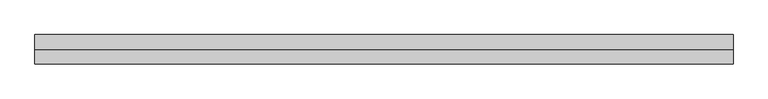
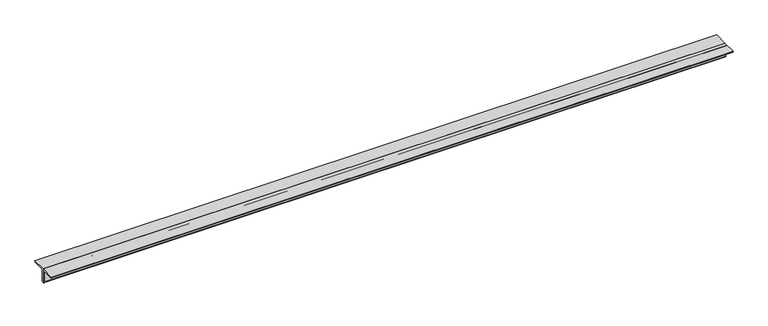
"""IFC4 building model written with IfcOpenShell, lengths in millimetres: member geometry, Steel Framing_2Ls_KS : H_SB_AR_S02_2Ls-100x100x10_VBR1."""

from ifc_helpers import new_model, si_unit, point, frame, frame_2d, origin, place, context, project, spatial, polyline, circle_curve, trimmed, segment, composite_curve, outline, extrude, source, transform, mapped, element, save


def member_d528801c(model_context):
    return source(origin(), model_context, "Body", "SweptSolid", [
        extrude(outline(composite_curve([segment(polyline([(0.0, 28.2), (100.0, 28.2)]), True, "CONTINUOUS"), segment(trimmed(circle_curve(frame_2d((90.0, 28.2)), 10.0), [point((100.0, 28.2))], [point((90.0, 18.2))], False, "CARTESIAN"), True, "CONTINUOUS"), segment(polyline([(90.0, 18.2), (20.0, 18.2)]), True, "CONTINUOUS"), segment(trimmed(circle_curve(frame_2d((20.0, 8.2)), 10.0), [point((20.0, 18.2))], [point((10.0, 8.2))], True, "CARTESIAN"), True, "CONTINUOUS"), segment(polyline([(10.0, 8.2), (10.0, -61.8)]), True, "CONTINUOUS"), segment(trimmed(circle_curve(frame_2d((0.0, -61.8)), 10.0), [point((10.0, -61.8))], [point((0.0, -71.8))], False, "CARTESIAN"), True, "CONTINUOUS"), segment(polyline([(0.0, -71.8), (0.0, 28.2)]), True, "CONTINUOUS")], self_intersect=False)), frame((-2590.3354834, 0.0, 0.0), z_axis=(1.0, 0.0, 0.0), x_axis=(0.0, 1.0, 0.0)), (0.0, 0.0, 1.0), 4755.0114784),
        extrude(outline(composite_curve([segment(polyline([(0.0, 28.2), (0.0, -71.8)]), True, "CONTINUOUS"), segment(trimmed(circle_curve(frame_2d((0.0, -61.8)), 10.0), [point((0.0, -71.8))], [point((-10.0, -61.8))], False, "CARTESIAN"), True, "CONTINUOUS"), segment(polyline([(-10.0, -61.8), (-10.0, 8.2)]), True, "CONTINUOUS"), segment(trimmed(circle_curve(frame_2d((-20.0, 8.2)), 10.0), [point((-10.0, 8.2))], [point((-20.0, 18.2))], True, "CARTESIAN"), True, "CONTINUOUS"), segment(polyline([(-20.0, 18.2), (-90.0, 18.2)]), True, "CONTINUOUS"), segment(trimmed(circle_curve(frame_2d((-90.0, 28.2)), 10.0), [point((-90.0, 18.2))], [point((-100.0, 28.2))], False, "CARTESIAN"), True, "CONTINUOUS"), segment(polyline([(-100.0, 28.2), (0.0, 28.2)]), True, "CONTINUOUS")], self_intersect=False)), frame((-2590.3354834, 0.0, 0.0), z_axis=(1.0, 0.0, 0.0), x_axis=(0.0, 1.0, 0.0)), (0.0, 0.0, 1.0), 4755.0114784),
    ])


if __name__ == "__main__":
    model = new_model("IFC4")
    model_context = context("Model", 3, world=origin())
    ifc_project = project(units=[si_unit("LENGTHUNIT", "METRE", prefix="MILLI")], contexts=[model_context])
    site = spatial("IfcSite", under=ifc_project)
    building = spatial("IfcBuilding", under=site)
    placement = place(None, origin())
    member_shape = member_d528801c(model_context)
    element("IfcMember", 1, ObjectType="Steel Framing_2Ls_KS : H_SB_AR_S02_2Ls-100x100x10_VBR1", at=placement, inside=building, context=model_context, shape_type="MappedRepresentation", body=[
        mapped(member_shape, transform((0.0, 0.0, 0.0), x_axis=(1.0, 0.0, 0.0), y_axis=(0.0, 1.0, 0.0), z_axis=(0.0, 0.0, 1.0))),
    ])
    save(model, "model.ifc")

# Revit data of these elements
# Type "Steel Framing_2Ls_KS : H_SB_AR_S02_2Ls-100x100x10_VBR1"
#   Type Comments = "MAIN"
#   Type Mark = "VBR1"
#   H_SectionID = "2Ls-100x100x10"
#   Assembly Code = "B10"
#   Legs = "LLBB"
#   H_Ratio for Additional Steel Plate = 0.2
#   W = 0
#   Perimeter = 0.80 m²/m
#   Nominal Weight = 29.80 kgf/m
#   Length [instance default] = 1524 mm
#   Space = 0 mm
#   b = 100 mm
#   d = 100 mm
#   t = 10 mm
#   y = 28.2 mm
#   A = 0.0038 m²
#   Structural Material [instance default] = Steel, 45-345
# Element 1 (IfcMember, "Steel Framing_2Ls_KS : H_SB_AR_S02_2Ls-100x100x10_VBR1")
#   Materials on its faces: "Steel, 45-345"
# Materials
#   "Steel, 45-345": class "Metal", colour RGB 189 187 185, transparency 0, Description = "Steel 345 MPa", Cost = 0
